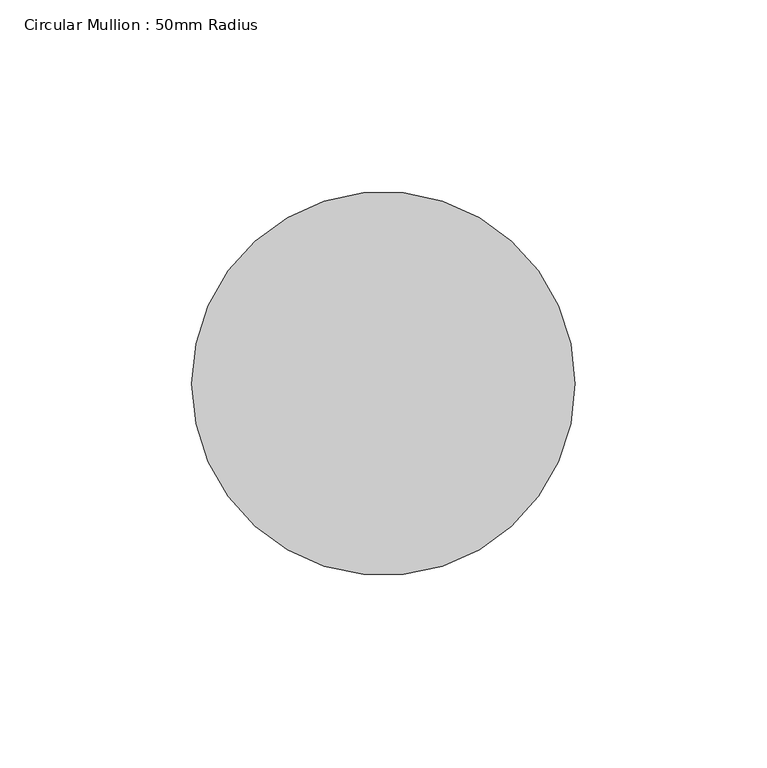
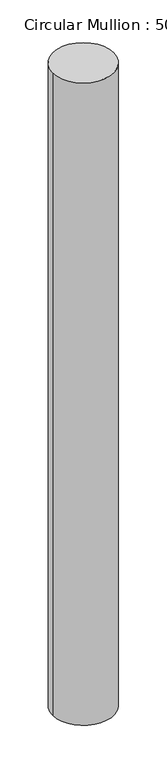
"""IFC4 building model written with IfcOpenShell, lengths in millimetres: member geometry, Circular Mullion : 50mm Radius."""

from ifc_helpers import new_model, si_unit, point, frame, origin, origin_2d, place, context, project, spatial, circle_curve, trimmed, segment, composite_curve, outline, extrude, source, transform, mapped, element, save


def circular_mullion_50mm_radius_01caa19f(model_context):
    return source(origin(), model_context, "Body", "SweptSolid", [
        extrude(outline(composite_curve([segment(trimmed(circle_curve(origin_2d(), 50.0), [point((50.0, 0.0))], [point((-50.0, 0.0))], False, "CARTESIAN"), True, "CONTINUOUS"), segment(trimmed(circle_curve(origin_2d(), 50.0), [point((-50.0, 0.0))], [point((50.0, 0.0))], False, "CARTESIAN"), True, "CONTINUOUS")], self_intersect=False)), frame((0.0, 0.0, -1114.3341279), z_axis=(0.0, 0.0, 1.0), x_axis=(1.0, 0.0, 0.0)), (0.0, 0.0, 1.0), 1114.3341279),
    ])


if __name__ == "__main__":
    model = new_model("IFC4")
    model_context = context("Model", 3, world=origin())
    ifc_project = project(units=[si_unit("LENGTHUNIT", "METRE", prefix="MILLI")], contexts=[model_context])
    site = spatial("IfcSite", under=ifc_project)
    building = spatial("IfcBuilding", under=site)
    placement = place(None, origin())
    circular_mullion_50mm_radius_shape = circular_mullion_50mm_radius_01caa19f(model_context)
    element("IfcMember", 1, ObjectType="Circular Mullion : 50mm Radius", at=placement, inside=building, context=model_context, shape_type="MappedRepresentation", body=[
        mapped(circular_mullion_50mm_radius_shape, transform((0.0, 0.0, 0.0), x_axis=(1.0, 0.0, 0.0), y_axis=(0.0, 1.0, 0.0), z_axis=(0.0, 0.0, 1.0))),
    ])
    save(model, "model.ifc")

# Revit data of these elements
# Type "Circular Mullion : 50mm Radius"
#   built-in parameter 1007350 = 0.164042 (stored number, unit not read)
# Element 1 (IfcMember, "Circular Mullion : 50mm Radius")
#   Materials on its faces: "Aluminium"
# Materials
#   "Aluminium": class "Metal", colour RGB 247 247 247, transparency 0, Description = "Aluminium 6061", Cost = 0
